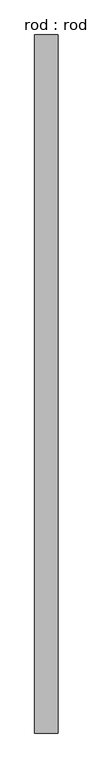
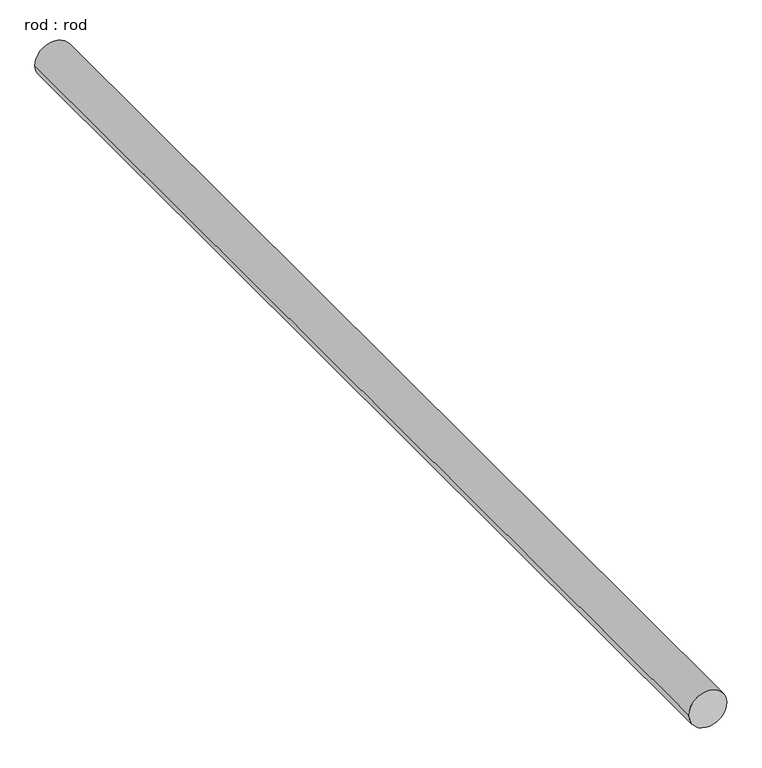
"""IFC4 building model written with IfcOpenShell, lengths in millimetres: proxy geometry, rod : rod."""

import ifcopenshell
import ifcopenshell.guid

model = None  # the IFC model being written
_history = None  # IfcOwnerHistory: only IFC2X3 demands one
_inside = {}  # id of a spatial element -> (the spatial element, [elements in it])
_under = {}  # id of a project, library or spatial element -> (it, [spatial elements below it])
_declared = {}  # id of a project -> (the project, [libraries it declares])
_typed = {}  # id of a type object -> (the type object, [elements of that type])
_made_of = {}  # id of a material, layer set ... -> (it, [elements and type objects made of it])


def new_model(schema):
    """Start an empty IFC model of exactly this schema.

    Asked for "IFC4X3", IfcOpenShell would pick the latest addendum, in which some entities
    have other attributes; the version numbers below select the first issue.
    IFC2X3 requires an IfcOwnerHistory on every rooted entity: one is made here for all.
    """
    global model, _history
    if schema == "IFC4X3":
        model = ifcopenshell.file(schema_version=(4, 3, 0, 0))
    else:
        model = ifcopenshell.file(schema=schema)
    _inside.clear()
    _under.clear()
    _declared.clear()
    _typed.clear()
    _made_of.clear()
    _history = None
    if model.schema == "IFC2X3":
        org = make("IfcOrganization", Name="unknown")
        user = make(
            "IfcPersonAndOrganization",
            ThePerson=make("IfcPerson", FamilyName="unknown"),
            TheOrganization=org,
        )
        app = make(
            "IfcApplication",
            ApplicationDeveloper=org,
            Version="unknown",
            ApplicationFullName="unknown",
            ApplicationIdentifier="unknown",
        )
        _history = make(
            "IfcOwnerHistory",
            OwningUser=user,
            OwningApplication=app,
            ChangeAction="ADDED",
            CreationDate=0,
        )
    return model


def make(cls, **values):
    """One entity of the class cls with the attributes given. An attribute that is None is left unset."""
    return model.create_entity(
        cls, **{name: value for name, value in values.items() if value is not None}
    )


def rooted(cls, **values):
    """An entity with a GlobalId (a new one), such as an element, a storey or a relation."""
    return make(cls, GlobalId=ifcopenshell.guid.new(), OwnerHistory=_history, **values)


def si_unit(unit_type, name, prefix=None):
    """IfcSIUnit, for example si_unit("LENGTHUNIT", "METRE", prefix="MILLI")."""
    return make("IfcSIUnit", UnitType=unit_type, Prefix=prefix, Name=name)


def assignment(units):
    """IfcUnitAssignment: the units of a project."""
    return None if units is None else make("IfcUnitAssignment", Units=units)


def point(xyz):
    """IfcCartesianPoint."""
    return None if xyz is None else make("IfcCartesianPoint", Coordinates=xyz)


def direction(xyz):
    """IfcDirection."""
    return None if xyz is None else make("IfcDirection", DirectionRatios=xyz)


def frame(location, z_axis=None, x_axis=None):
    """IfcAxis2Placement3D, a coordinate frame: its origin and axes. An axis left out is left unset."""
    return make(
        "IfcAxis2Placement3D",
        Location=point(location),
        Axis=direction(z_axis),
        RefDirection=direction(x_axis),
    )


def frame_2d(location, x_axis=None):
    """IfcAxis2Placement2D, a coordinate frame in the plane: its origin and x axis."""
    return make(
        "IfcAxis2Placement2D", Location=point(location), RefDirection=direction(x_axis)
    )


def origin():
    """The frame at (0, 0, 0) with its axes left unset."""
    return frame((0.0, 0.0, 0.0))


def place(relative_to, where):
    """IfcLocalPlacement: puts the frame where relative to a parent placement (None: the world)."""
    return make(
        "IfcLocalPlacement", PlacementRelTo=relative_to, RelativePlacement=where
    )


def context(
    kind, dimensions, precision=None, world=None, true_north=None, identifier=None
):
    """IfcGeometricRepresentationContext, for example the 3D "Model" context."""
    return make(
        "IfcGeometricRepresentationContext",
        ContextIdentifier=identifier,
        ContextType=kind,
        CoordinateSpaceDimension=dimensions,
        Precision=precision,
        WorldCoordinateSystem=world,
        TrueNorth=true_north,
    )


def project(units=None, contexts=None):
    """IfcProject with its units and contexts."""
    return rooted(
        "IfcProject",
        Name="project",
        RepresentationContexts=contexts,
        UnitsInContext=assignment(units),
    )


def spatial(cls, under=None, at=None, **own):
    """A site, building, storey or space (cls), placed at a placement, below another one or the project."""
    s = rooted(cls, ObjectPlacement=at, **own)
    if under is not None:
        _under.setdefault(under.id(), (under, []))[1].append(s)
    return s


def circle_curve(where, radius):
    """IfcCircle in the frame where."""
    return make("IfcCircle", Position=where, Radius=radius)


def trimmed(basis, trim1, trim2, sense, master):
    """IfcTrimmedCurve: the piece of a basis curve between two trims."""
    return make(
        "IfcTrimmedCurve",
        BasisCurve=basis,
        Trim1=trim1,
        Trim2=trim2,
        SenseAgreement=sense,
        MasterRepresentation=master,
    )


def segment(curve, same_sense, transition):
    """IfcCompositeCurveSegment."""
    return make(
        "IfcCompositeCurveSegment",
        Transition=transition,
        SameSense=same_sense,
        ParentCurve=curve,
    )


def composite_curve(segments, self_intersect=None):
    """IfcCompositeCurve: segments joined end to end."""
    return make("IfcCompositeCurve", Segments=segments, SelfIntersect=self_intersect)


def outline(outer, holes=None, kind="AREA"):
    """IfcArbitraryClosedProfileDef: a profile drawn as a closed curve; with holes, ...WithVoids."""
    if holes is None:
        return make("IfcArbitraryClosedProfileDef", ProfileType=kind, OuterCurve=outer)
    return make(
        "IfcArbitraryProfileDefWithVoids",
        ProfileType=kind,
        OuterCurve=outer,
        InnerCurves=holes,
    )


def extrude(swept, where, along, depth):
    """IfcExtrudedAreaSolid: the profile swept, set in the frame where, extruded along a direction by depth."""
    return make(
        "IfcExtrudedAreaSolid",
        SweptArea=swept,
        Position=where,
        ExtrudedDirection=direction(along),
        Depth=depth,
    )


def shape(context_of_items, identifier, shape_type, items):
    """IfcShapeRepresentation: the items that make up one representation, for example the "Body"."""
    return make(
        "IfcShapeRepresentation",
        ContextOfItems=context_of_items,
        RepresentationIdentifier=identifier,
        RepresentationType=shape_type,
        Items=items,
    )


def source(mapping_origin, context_of_items, identifier, shape_type, items):
    """IfcRepresentationMap: a shape defined once, which mapped items show again and again."""
    return make(
        "IfcRepresentationMap",
        MappingOrigin=mapping_origin,
        MappedRepresentation=shape(context_of_items, identifier, shape_type, items),
    )


def transform(
    local_origin,
    x_axis=None,
    y_axis=None,
    z_axis=None,
    scale=None,
    scale2=None,
    scale3=None,
    uniform=True,
):
    """IfcCartesianTransformationOperator3D, or its non-uniform kind. x_axis, y_axis, z_axis: its Axis1, 2, 3."""
    if uniform:
        return make(
            "IfcCartesianTransformationOperator3D",
            Axis1=direction(x_axis),
            Axis2=direction(y_axis),
            LocalOrigin=point(local_origin),
            Scale=scale,
            Axis3=direction(z_axis),
        )
    return make(
        "IfcCartesianTransformationOperator3DnonUniform",
        Axis1=direction(x_axis),
        Axis2=direction(y_axis),
        LocalOrigin=point(local_origin),
        Scale=scale,
        Axis3=direction(z_axis),
        Scale2=scale2,
        Scale3=scale3,
    )


def mapped(mapping_source, mapping_target):
    """IfcMappedItem: shows the shape of a source again, moved by a transform."""
    return make(
        "IfcMappedItem", MappingSource=mapping_source, MappingTarget=mapping_target
    )


def made_of(thing, what):
    """Note that an element or type object is made of a material, layer set ...; save() writes the relation."""
    if what is not None:
        _made_of.setdefault(what.id(), (what, []))[1].append(thing)
    return thing


def element(
    cls,
    number,
    at=None,
    inside=None,
    cuts=None,
    type_object=None,
    material=None,
    context=None,
    identifier="Body",
    shape_type=None,
    held_by="IfcProductDefinitionShape",
    body=None,
    shapes=None,
    **own,
):
    """One element of the class cls, such as IfcWall. Its Tag is "e" and its number.

    at: its placement. inside: the storey or other place that contains it. cuts: it is an
    opening in that element (IfcRelVoidsElement). A single representation is given by context,
    identifier, shape_type and body (its items); several are given by shapes. held_by: the class
    of the entity that holds the representations. save() writes the other relations.
    """
    e = rooted(cls, Tag="e%d" % number, ObjectPlacement=at, **own)
    if body is not None:
        shapes = [shape(context, identifier, shape_type, body)]
    if shapes is not None:
        e.Representation = make(held_by, Representations=shapes)
    if inside is not None:
        _inside.setdefault(inside.id(), (inside, []))[1].append(e)
    if cuts is not None:
        rooted(
            "IfcRelVoidsElement", RelatingBuildingElement=cuts, RelatedOpeningElement=e
        )
    if type_object is not None:
        _typed.setdefault(type_object.id(), (type_object, []))[1].append(e)
    return made_of(e, material)


def aggregate(whole, parts):
    """IfcRelAggregates: a whole, such as a stair, and the parts it consists of."""
    return rooted("IfcRelAggregates", RelatingObject=whole, RelatedObjects=parts)


def save(model, path):
    """Write the relations noted so far, then the file.

    IfcRelAggregates (storeys below a building ...), IfcRelContainedInSpatialStructure (elements
    in a storey), IfcRelDefinesByType, IfcRelAssociatesMaterial and IfcRelDeclares: one each for
    every whole, place, type object, material and project.
    """
    for whole, parts in _under.values():
        aggregate(whole, parts)
    for where, things in _inside.values():
        rooted(
            "IfcRelContainedInSpatialStructure",
            RelatedElements=things,
            RelatingStructure=where,
        )
    for kind, things in _typed.values():
        rooted("IfcRelDefinesByType", RelatedObjects=things, RelatingType=kind)
    for what, things in _made_of.values():
        rooted("IfcRelAssociatesMaterial", RelatedObjects=things, RelatingMaterial=what)
    for by, libraries in _declared.values():
        rooted("IfcRelDeclares", RelatingContext=by, RelatedDefinitions=libraries)
    model.write(path)


def rod_rod_c9aaecbc(model_context):
    return source(origin(), model_context, "Body", "SweptSolid", [
        extrude(outline(composite_curve([segment(trimmed(circle_curve(frame_2d((0.0108462, 0.0)), 200.0), [point((0.0108462, 200.0))], [point((0.0108462, -200.0))], False, "CARTESIAN"), True, "CONTINUOUS"), segment(trimmed(circle_curve(frame_2d((0.0108462, 0.0)), 200.0), [point((0.0108462, -200.0))], [point((0.0108462, 200.0))], False, "CARTESIAN"), True, "CONTINUOUS")], self_intersect=False)), frame((0.0, -1854.4319791, 0.0), z_axis=(0.0, 1.0, 0.0), x_axis=(0.0, 0.0, 1.0)), (0.0, 0.0, 1.0), 11894.3211888),
    ])


if __name__ == "__main__":
    model = new_model("IFC4")
    model_context = context("Model", 3, world=origin())
    ifc_project = project(units=[si_unit("LENGTHUNIT", "METRE", prefix="MILLI")], contexts=[model_context])
    site = spatial("IfcSite", under=ifc_project)
    building = spatial("IfcBuilding", under=site)
    placement = place(None, origin())
    rod_rod_shape = rod_rod_c9aaecbc(model_context)
    element("IfcBuildingElementProxy", 1, Name="rod : rod", ObjectType="rod : rod", at=placement, inside=building, context=model_context, shape_type="MappedRepresentation", body=[
        mapped(rod_rod_shape, transform((0.0, 0.0, 0.0), x_axis=(1.0, 0.0, 0.0), y_axis=(0.0, 1.0, 0.0), z_axis=(0.0, 0.0, 1.0))),
    ])
    save(model, "model.ifc")

# Revit data of these elements
# Type "rod : rod"
#   Default Elevation = 0
